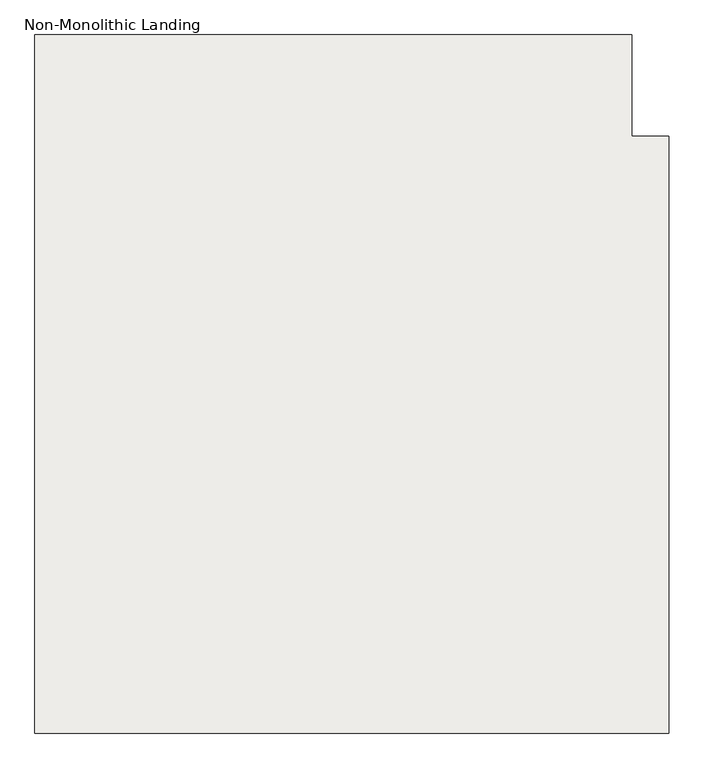
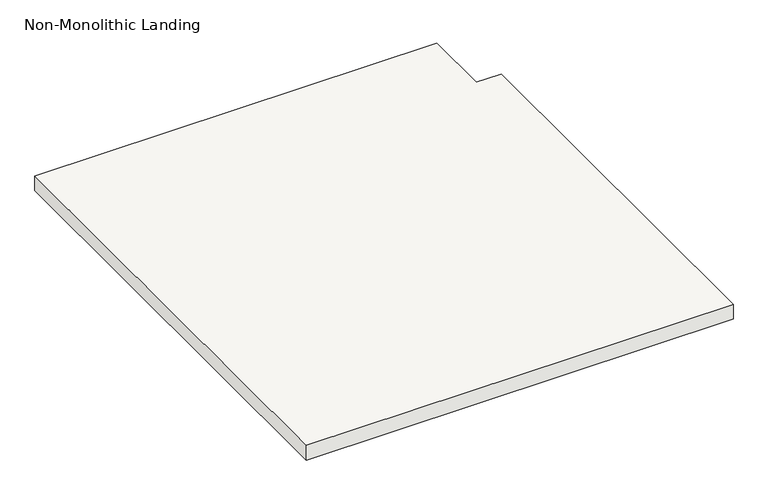
"""IFC4 building model written with IfcOpenShell, lengths in millimetres: slab geometry, Non-Monolithic Landing."""

from ifc_helpers import new_model, si_unit, frame, origin, place, context, project, spatial, polyline, outline, extrude, source, transform, mapped, element, save


def non_monolithic_landing_63f0f0fd(model_context):
    return source(origin(), model_context, "Body", "SweptSolid", [
        extrude(outline(polyline([(-13195.5859635, -3521.1593564), (-14576.101437, -3521.1593564), (-14576.101437, -2000.1378151), (-13276.101437, -2000.1378151), (-13276.101437, -2221.1593564), (-13195.5859635, -2221.1593564), (-13195.5859635, -3521.1593564)])), frame((0.0, 0.0, 1450.0), z_axis=(0.0, 0.0, 1.0), x_axis=(1.0, 0.0, 0.0)), (0.0, 0.0, 1.0), 50.0),
    ])


if __name__ == "__main__":
    model = new_model("IFC4")
    model_context = context("Model", 3, world=origin())
    ifc_project = project(units=[si_unit("LENGTHUNIT", "METRE", prefix="MILLI")], contexts=[model_context])
    site = spatial("IfcSite", under=ifc_project)
    building = spatial("IfcBuilding", under=site)
    placement = place(None, origin())
    non_monolithic_landing_shape = non_monolithic_landing_63f0f0fd(model_context)
    element("IfcSlab", 1, ObjectType="Non-Monolithic Landing", at=placement, inside=building, context=model_context, shape_type="MappedRepresentation", body=[
        mapped(non_monolithic_landing_shape, transform((0.0, 0.0, 0.0), x_axis=(1.0, 0.0, 0.0), y_axis=(0.0, 1.0, 0.0), z_axis=(0.0, 0.0, 1.0))),
    ])
    save(model, "model.ifc")
